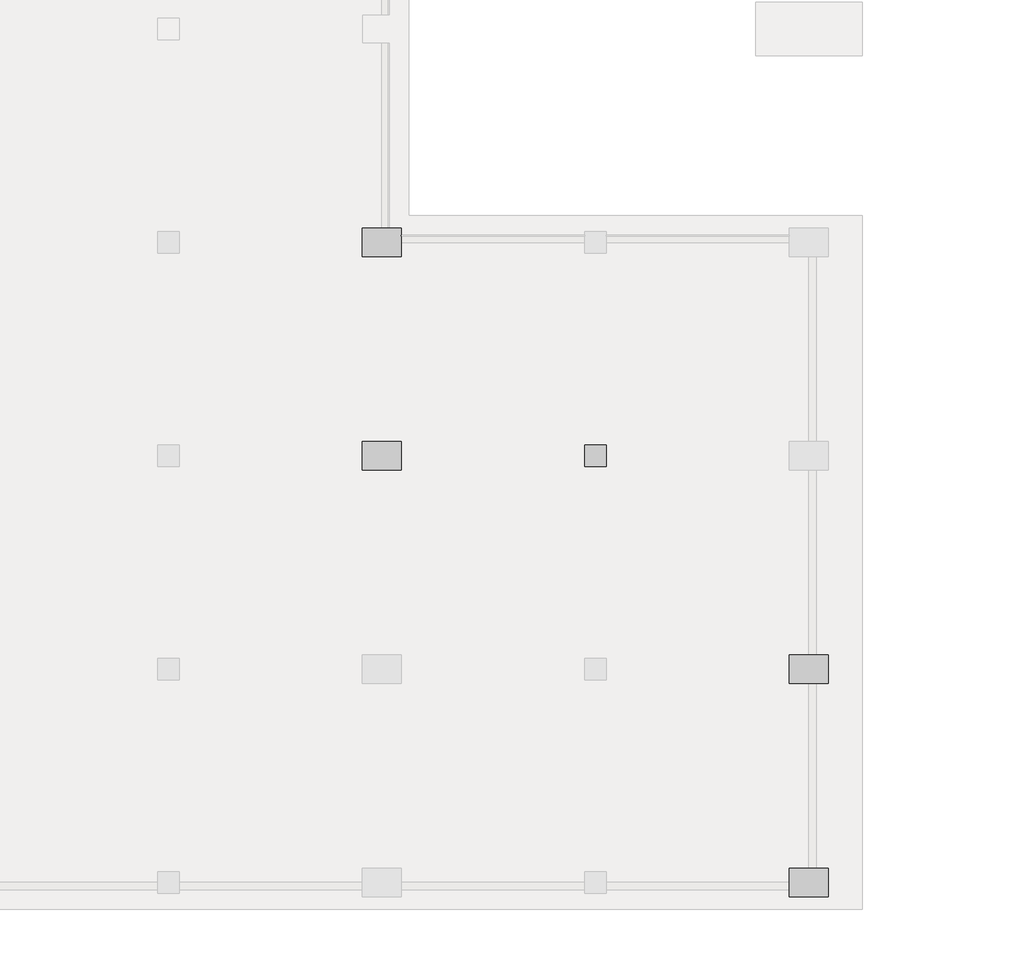
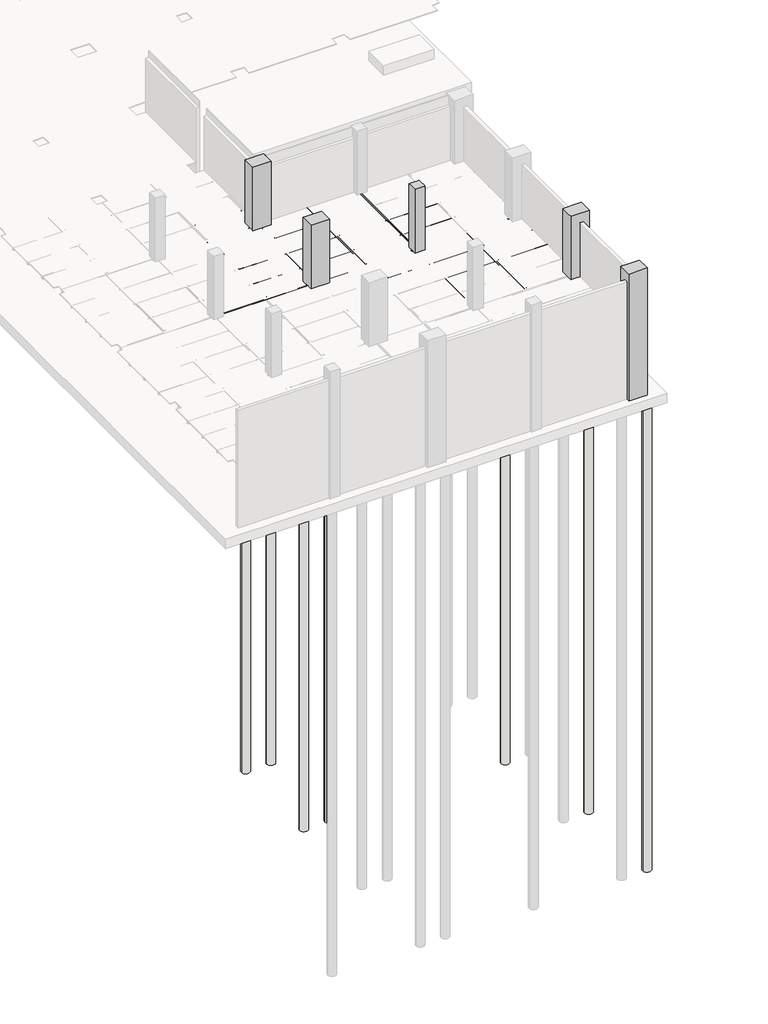
# Not in any storey, part 5 of 16: 26 beams, 7 slabs, 5 columns.
# Revit data of these elements (continued)
# Element 31 (IfcColumn, "RC_Column_Rectangular : H_SC_AR_S15_UG PED_Bit_600x600_BC1") (continued)
#   Materials on its faces: "00_Concrete_Reinf. Conc."
# Elements 32, 33, 34, 35, 36, 37, 38 (IfcSlab, "PILE : H_SF_AR_S19_PHC Pile_Pre-boring_D500_L30")
#   Structural Material = none
#   Phase Created = New Construction
# Materials
#   "Steel, 45-345": class "Metal", colour RGB 189 187 185, transparency 0, Description = "Steel 345 MPa", Cost = 0
#   "00_Concrete_Reinf. Conc.": class "Concrete", colour RGB 176 176 176, transparency 0, Description = "Reinf. Conc.", Cost = 0, Image = Concrete.Cast-In-Place.Flat.Polished.Grey.jpg
